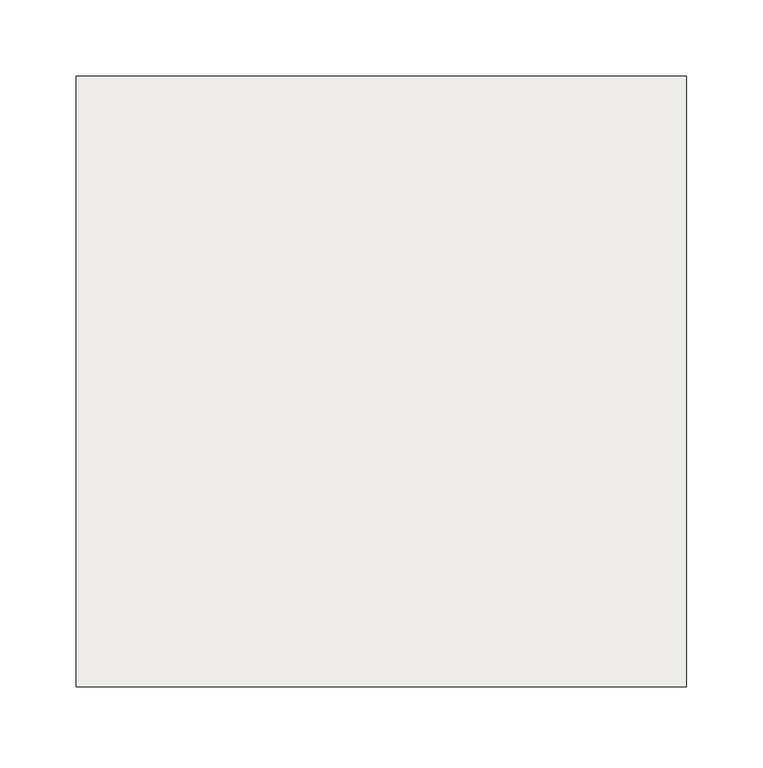
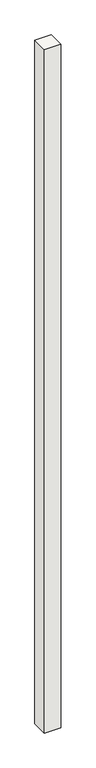
"""IFC4 building model written with IfcOpenShell, lengths in millimetres: footing geometry, NLRS_17_SFO_TLB_funderingspaal geheid beton prefab-AV-MMBPC_gen_rsf : heipaal beton prefab_gen__bxh 400x400."""

from ifc_helpers import new_model, si_unit, frame, origin, place, context, project, spatial, polyline, outline, extrude, source, transform, mapped, element, save


def footing_f6128070(model_context):
    return source(origin(), model_context, "Body", "SweptSolid", [
        extrude(outline(polyline([(200.0, -200.0), (-200.0, -200.0), (-200.0, 200.0), (200.0, 200.0), (200.0, -200.0)])), frame((0.0, 0.0, -20000.0), z_axis=(0.0, 0.0, 1.0), x_axis=(1.0, 0.0, 0.0)), (0.0, 0.0, 1.0), 17610.0),
    ])


if __name__ == "__main__":
    model = new_model("IFC4")
    model_context = context("Model", 3, world=origin())
    ifc_project = project(units=[si_unit("LENGTHUNIT", "METRE", prefix="MILLI")], contexts=[model_context])
    site = spatial("IfcSite", under=ifc_project)
    building = spatial("IfcBuilding", under=site)
    placement = place(None, origin())
    footing_shape = footing_f6128070(model_context)
    element("IfcFooting", 1, ObjectType="NLRS_17_SFO_TLB_funderingspaal geheid beton prefab-AV-MMBPC_gen_rsf : heipaal beton prefab_gen__bxh 400x400", at=placement, inside=building, context=model_context, shape_type="MappedRepresentation", body=[
        mapped(footing_shape, transform((0.0, 0.0, 0.0), x_axis=(1.0, 0.0, 0.0), y_axis=(0.0, 1.0, 0.0), z_axis=(0.0, 0.0, 1.0))),
    ])
    save(model, "model.ifc")

# Revit data of these elements
# Type "NLRS_17_SFO_TLB_funderingspaal geheid beton prefab-AV-MMBPC_gen_rsf : heipaal beton prefab_gen__bxh 400x400"
#   IfcExportAs = "IfcPile"
#   Type Comments = "prefab heipaal 400x400"
#   Model = " "
#   Manufacturer = " "
#   Description = "prefab heipaal 400x400"
#   Assembly Code = "17.21"
#   Width = 400 mm
#   Slanted Angle [instance default] = 0.00°
#   NLRS_S_draagvermogen_trek [instance default] = 0.00 kN
#   NLRS_S_draagvermogen_druk [instance default] = 0.00 kN
#   NLRS_C_lengte [instance default] = 1660 mm
#   NLRS_C_hoogte = 400 mm
#   NLRS_C_breedte = 400 mm
#   Height [instance default] = 1660 mm
#   Length [instance default] = 1660 mm
#   Angle [instance default] = 0.00°
#   Slanted [instance default] = 0
#   Structural Material = NLRS_f2_beton prefab_gen_rsf
#   Keynote = ""
# Element 1 (IfcFooting, "NLRS_17_SFO_TLB_funderingspaal geheid beton prefab-AV-MMBPC_gen_rsf : heipaal beton prefab_gen__bxh 400x400")
#   NLRS_C_lengte = 17610 mm
#   Height = 17610 mm
#   Length = 17610 mm
#   Materials on its faces: "NLRS_f2_beton prefab_gen_rsf"
# Materials
#   "NLRS_f2_beton prefab_gen_rsf": class "F - Niet gebakken kunststeen", colour RGB 129 133 118, transparency 0, Keynote = "f2", Manufacturer = "Revit Standards Foundation", URL = "www.revitstandards.org", Description = "beton prefab", Cost = 0
